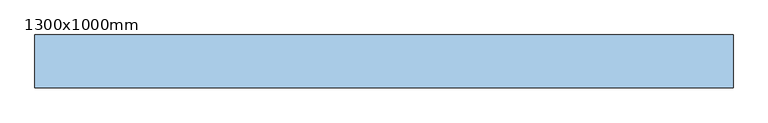
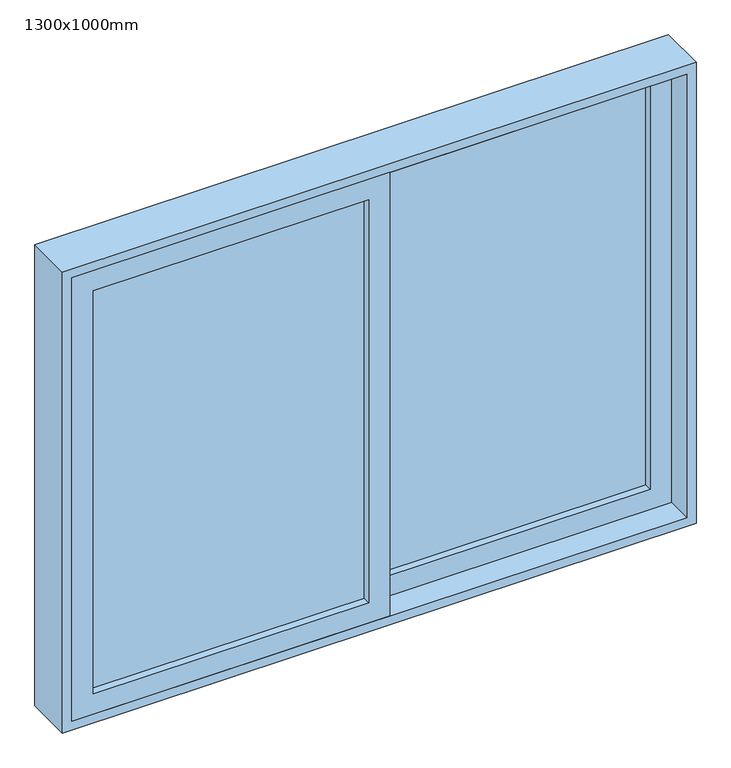
"""IFC4 building model written with IfcOpenShell, lengths in millimetres: window geometry, Janela de Correr - 2 Folhas : 1300x1000mm."""

from ifc_helpers import new_model, si_unit, frame, origin, place, context, project, spatial, polyline, outline, extrude, source, transform, mapped, element, save


def window_1300x1000mm_a11e05bc(model_context):
    return source(origin(), model_context, "Body", "SweptSolid", [
        extrude(outline(polyline([(-587.0, -44.6), (-22.0, -44.6), (-22.0, -56.6), (-587.0, -56.6), (-587.0, -44.6)])), frame((0.0, 0.0, 1263.0), z_axis=(0.0, 0.0, 1.0), x_axis=(1.0, 0.0, 0.0)), (0.0, 0.0, 1.0), 874.0),
        extrude(outline(polyline([(2181.0, 22.0), (2181.0, -631.0), (1219.0, -631.0), (1219.0, 22.0), (2181.0, 22.0)]), holes=[polyline([(2137.0, -22.0), (1263.0, -22.0), (1263.0, -587.0), (2137.0, -587.0), (2137.0, -22.0)])]), frame((0.0, -72.6, 0.0), z_axis=(0.0, 1.0, 0.0), x_axis=(0.0, 0.0, 1.0)), (0.0, 0.0, 1.0), 44.0),
        extrude(outline(polyline([(22.0, 9.4), (587.0, 9.4), (587.0, -2.6), (22.0, -2.6), (22.0, 9.4)])), frame((0.0, 0.0, 1263.0), z_axis=(0.0, 0.0, 1.0), x_axis=(1.0, 0.0, 0.0)), (0.0, 0.0, 1.0), 874.0),
        extrude(outline(polyline([(2181.0, -22.0), (1219.0, -22.0), (1219.0, 631.0), (2181.0, 631.0), (2181.0, -22.0)]), holes=[polyline([(2137.0, 22.0), (2137.0, 587.0), (1263.0, 587.0), (1263.0, 22.0), (2137.0, 22.0)])]), frame((0.0, -18.6, 0.0), z_axis=(0.0, 1.0, 0.0), x_axis=(0.0, 0.0, 1.0)), (0.0, 0.0, 1.0), 44.0),
        extrude(outline(polyline([(2200.0, -650.0), (1200.0, -650.0), (1200.0, 650.0), (2200.0, 650.0), (2200.0, -650.0)]), holes=[polyline([(2181.0, -631.0), (2181.0, 631.0), (1219.0, 631.0), (1219.0, -631.0), (2181.0, -631.0)])]), frame((0.0, -72.6, 0.0), z_axis=(0.0, 1.0, 0.0), x_axis=(0.0, 0.0, 1.0)), (0.0, 0.0, 1.0), 98.0),
    ])


if __name__ == "__main__":
    model = new_model("IFC4")
    model_context = context("Model", 3, world=origin())
    ifc_project = project(units=[si_unit("LENGTHUNIT", "METRE", prefix="MILLI")], contexts=[model_context])
    site = spatial("IfcSite", under=ifc_project)
    building = spatial("IfcBuilding", under=site)
    placement = place(None, origin())
    window_1300x1000mm_shape = window_1300x1000mm_a11e05bc(model_context)
    element("IfcWindow", 1, ObjectType="Janela de Correr - 2 Folhas : 1300x1000mm", at=placement, inside=building, context=model_context, shape_type="MappedRepresentation", body=[
        mapped(window_1300x1000mm_shape, transform((0.0, 0.0, 0.0), x_axis=(1.0, 0.0, 0.0), y_axis=(0.0, 1.0, 0.0), z_axis=(0.0, 0.0, 1.0))),
    ])
    save(model, "model.ifc")

# Revit data of these elements
# Type "Janela de Correr - 2 Folhas : 1300x1000mm"
#   Type Mark = "J1"
#   SINAPI = ""
#   Módulo Básico M = 10.00 cm
#   Largura de Coordenação Modular CM = 130.00 cm
#   Altura de Coordenação Modular CM = 100.00 cm
#   Height = 100.00 cm
#   Altura Peitoril = 120.00 cm
#   Width = 130.00 cm
#   Largura Marco = 1.90 cm
#   Número de Módulos Básicos nM Largura = 13
#   Número de Módulos Básicos nM Altura = 10
#   Material Marco = Metal - Alumínio
#   Material Vidro = Vidro
#   Material Perfil = Metal - Alumínio
#   Construction Type = (empty or 0)
#   Description = (empty or 0)
#   Assembly Code = ""
#   Wall Closure = (empty or 0)
# Element 1 (IfcWindow, "Janela de Correr - 2 Folhas : 1300x1000mm")
#   Materials on its faces: "Metal - Alumínio", "Vidro", "Madeira - Faixa"
# Materials
#   "Metal - Alumínio": class "Metal", colour RGB 244 244 244, transparency 0
#   "Vidro": class "Vidro", colour RGB 230 230 230, transparency 0.75, Cost = 0
#   "Madeira - Faixa": class "Madeira", colour RGB 107 81 55, transparency 0, Cost = 0
